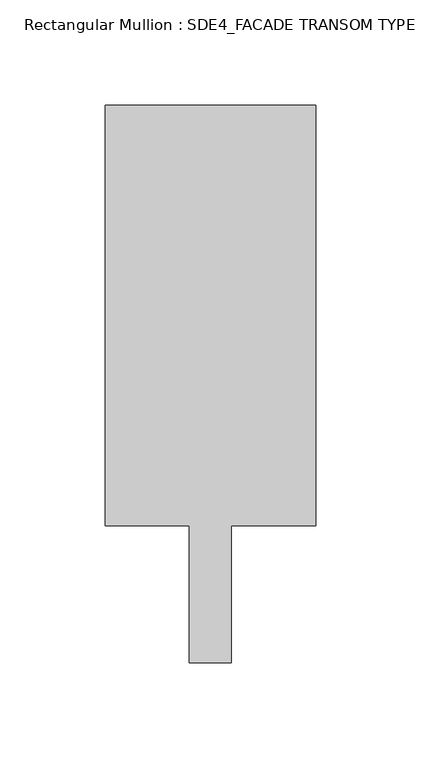
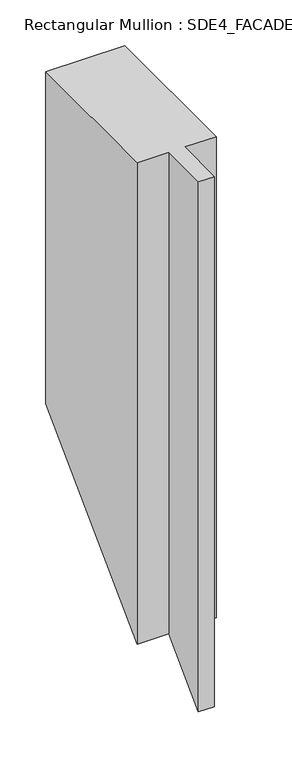
"""IFC4 building model written with IfcOpenShell, lengths in millimetres: member geometry, Rectangular Mullion : SDE4_FACADE TRANSOM TYPE 2."""

from ifc_helpers import new_model, si_unit, origin, place, context, project, spatial, faceted_brep, source, transform, mapped, element, save


def rectangular_mullion_sde4_facade_transom_type_2_174ae088(model_context):
    return source(origin(), model_context, "Body", "Brep", [
        faceted_brep([(50.0, 132.5, 0.0), (-50.0, 132.5, 0.0), (-50.0, -67.5, 0.0), (-10.0, -67.5, 0.0), (-10.0, -132.5, 0.0), (10.0, -132.5, 0.0), (10.0, -67.5, 0.0), (50.0, -67.5, 0.0), (50.0, 132.5, -442.9475465), (-50.0, 132.5, -442.9475465), (-50.0, -67.5, -642.9475465), (-10.0, -67.5, -642.9475465), (-10.0, -132.5, -707.9475465), (10.0, -132.5, -707.9475465), (10.0, -67.5, -642.9475465), (50.0, -67.5, -642.9475465)], [[[0, 1, 2, 3, 4, 5, 6, 7]], [[1, 0, 8, 9]], [[2, 1, 9, 10]], [[3, 2, 10, 11]], [[4, 3, 11, 12]], [[5, 4, 12, 13]], [[6, 5, 13, 14]], [[7, 6, 14, 15]], [[0, 7, 15, 8]], [[8, 15, 14, 13, 12, 11, 10, 9]]]),
    ])


if __name__ == "__main__":
    model = new_model("IFC4")
    model_context = context("Model", 3, world=origin())
    ifc_project = project(units=[si_unit("LENGTHUNIT", "METRE", prefix="MILLI")], contexts=[model_context])
    site = spatial("IfcSite", under=ifc_project)
    building = spatial("IfcBuilding", under=site)
    placement = place(None, origin())
    rectangular_mullion_sde4_facade_transom_type_2_shape = rectangular_mullion_sde4_facade_transom_type_2_174ae088(model_context)
    element("IfcMember", 1, ObjectType="Rectangular Mullion : SDE4_FACADE TRANSOM TYPE 2", at=placement, inside=building, context=model_context, shape_type="MappedRepresentation", body=[
        mapped(rectangular_mullion_sde4_facade_transom_type_2_shape, transform((0.0, 0.0, 0.0), x_axis=(1.0, 0.0, 0.0), y_axis=(0.0, 1.0, 0.0), z_axis=(0.0, 0.0, 1.0))),
    ])
    save(model, "model.ifc")

# Revit data of these elements
# Type "Rectangular Mullion : SDE4_FACADE TRANSOM TYPE 2"
#   built-in parameter 1007322 = 0.869423 (stored number, unit not read)
#   built-in parameter 1007321 = 0.164042 (stored number, unit not read)
#   built-in parameter 1007320 = 0.164042 (stored number, unit not read)
